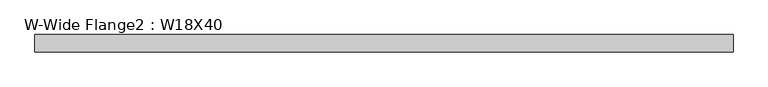
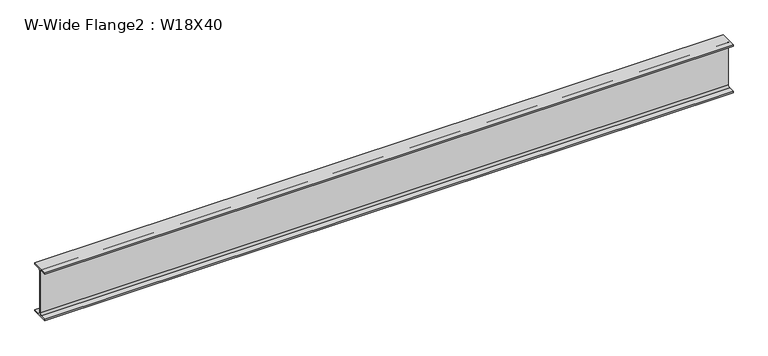
"""IFC4 building model written with IfcOpenShell, lengths in millimetres: beam geometry, W-Wide Flange2 : W18X40."""

from ifc_helpers import new_model, si_unit, point, frame, frame_2d, origin, place, context, project, spatial, polyline, circle_curve, trimmed, segment, composite_curve, outline, extrude, source, transform, mapped, element, save


def w_wide_flange2_w18x40_30b59f7b(model_context):
    return source(origin(), model_context, "Body", "SweptSolid", [
        extrude(outline(composite_curve([segment(polyline([(76.454, -213.995), (76.454, -227.33), (-76.454, -227.33), (-76.454, -213.995), (-20.828, -213.995)]), True, "CONTINUOUS"), segment(trimmed(circle_curve(frame_2d((-20.828, -197.1675)), 16.8275), [point((-20.828, -213.995))], [point((-4.0005, -197.1675))], True, "CARTESIAN"), True, "CONTINUOUS"), segment(polyline([(-4.0005, -197.1675), (-4.0005, 197.1675)]), True, "CONTINUOUS"), segment(trimmed(circle_curve(frame_2d((-20.828, 197.1675)), 16.8275), [point((-4.0005, 197.1675))], [point((-20.828, 213.995))], True, "CARTESIAN"), True, "CONTINUOUS"), segment(polyline([(-20.828, 213.995), (-76.454, 213.995), (-76.454, 227.33), (76.454, 227.33), (76.454, 213.995), (20.828, 213.995)]), True, "CONTINUOUS"), segment(trimmed(circle_curve(frame_2d((20.828, 197.1675)), 16.8275), [point((20.828, 213.995))], [point((4.0005, 197.1675))], True, "CARTESIAN"), True, "CONTINUOUS"), segment(polyline([(4.0005, 197.1675), (4.0005, -197.1675)]), True, "CONTINUOUS"), segment(trimmed(circle_curve(frame_2d((20.828, -197.1675)), 16.8275), [point((4.0005, -197.1675))], [point((20.828, -213.995))], True, "CARTESIAN"), True, "CONTINUOUS"), segment(polyline([(20.828, -213.995), (76.454, -213.995)]), True, "CONTINUOUS")], self_intersect=False)), frame((-3079.353125, 0.0, 0.0), z_axis=(1.0, 0.0, 0.0), x_axis=(0.0, 1.0, 0.0)), (0.0, 0.0, 1.0), 6158.70625),
    ])


if __name__ == "__main__":
    model = new_model("IFC4")
    model_context = context("Model", 3, world=origin())
    ifc_project = project(units=[si_unit("LENGTHUNIT", "METRE", prefix="MILLI")], contexts=[model_context])
    site = spatial("IfcSite", under=ifc_project)
    building = spatial("IfcBuilding", under=site)
    placement = place(None, origin())
    w_wide_flange2_w18x40_shape = w_wide_flange2_w18x40_30b59f7b(model_context)
    element("IfcBeam", 1, ObjectType="W-Wide Flange2 : W18X40", at=placement, inside=building, context=model_context, shape_type="MappedRepresentation", body=[
        mapped(w_wide_flange2_w18x40_shape, transform((0.0, 0.0, 0.0), x_axis=(1.0, 0.0, 0.0), y_axis=(0.0, 1.0, 0.0), z_axis=(0.0, 0.0, 1.0))),
    ])
    save(model, "model.ifc")

# Revit data of these elements
# Type "W-Wide Flange2 : W18X40"
#   Assembly Code = "B10"
#   W = 40
#   Length [instance default] = 5' - 0"
#   bf = 0' - 6.02"
#   d = 1' - 5.9"
#   k = 0' - 1 3/16"
#   k2 = 0' - 0.6625"
#   tf = 0' - 0.525"
#   tw = 0' - 0.315"
#   A = 0.0819444 SF
#   Structural Material [instance default] = Steel ASTM A992
# Element 1 (IfcBeam, "W-Wide Flange2 : W18X40")
#   Materials on its faces: "Steel ASTM A992"
# Materials
#   "Steel ASTM A992": class "Metal", colour RGB 199 199 199, transparency 0, Description = "Structural steel 50ksi", Cost = 0
